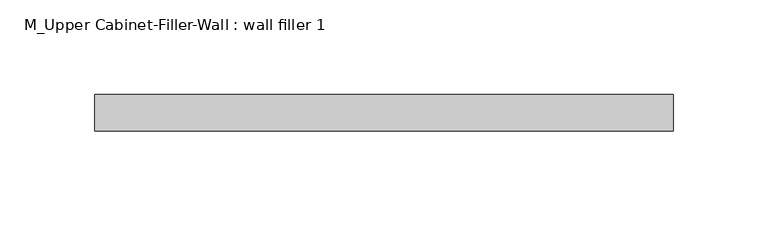
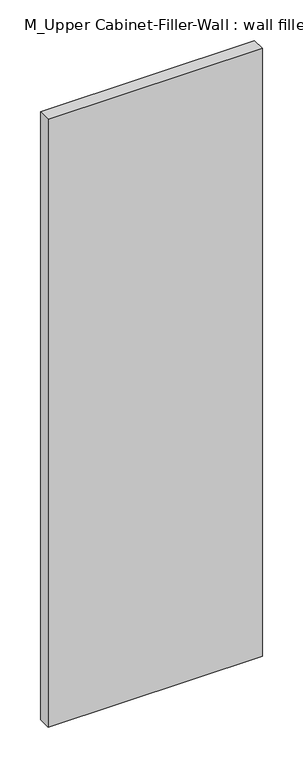
"""IFC4 building model written with IfcOpenShell, lengths in millimetres: furniture geometry, M_Upper Cabinet-Filler-Wall : wall filler 1."""

import ifcopenshell
import ifcopenshell.guid

model = None  # the IFC model being written
_history = None  # IfcOwnerHistory: only IFC2X3 demands one
_inside = {}  # id of a spatial element -> (the spatial element, [elements in it])
_under = {}  # id of a project, library or spatial element -> (it, [spatial elements below it])
_declared = {}  # id of a project -> (the project, [libraries it declares])
_typed = {}  # id of a type object -> (the type object, [elements of that type])
_made_of = {}  # id of a material, layer set ... -> (it, [elements and type objects made of it])


def new_model(schema):
    """Start an empty IFC model of exactly this schema.

    Asked for "IFC4X3", IfcOpenShell would pick the latest addendum, in which some entities
    have other attributes; the version numbers below select the first issue.
    IFC2X3 requires an IfcOwnerHistory on every rooted entity: one is made here for all.
    """
    global model, _history
    if schema == "IFC4X3":
        model = ifcopenshell.file(schema_version=(4, 3, 0, 0))
    else:
        model = ifcopenshell.file(schema=schema)
    _inside.clear()
    _under.clear()
    _declared.clear()
    _typed.clear()
    _made_of.clear()
    _history = None
    if model.schema == "IFC2X3":
        org = make("IfcOrganization", Name="unknown")
        user = make(
            "IfcPersonAndOrganization",
            ThePerson=make("IfcPerson", FamilyName="unknown"),
            TheOrganization=org,
        )
        app = make(
            "IfcApplication",
            ApplicationDeveloper=org,
            Version="unknown",
            ApplicationFullName="unknown",
            ApplicationIdentifier="unknown",
        )
        _history = make(
            "IfcOwnerHistory",
            OwningUser=user,
            OwningApplication=app,
            ChangeAction="ADDED",
            CreationDate=0,
        )
    return model


def make(cls, **values):
    """One entity of the class cls with the attributes given. An attribute that is None is left unset."""
    return model.create_entity(
        cls, **{name: value for name, value in values.items() if value is not None}
    )


def rooted(cls, **values):
    """An entity with a GlobalId (a new one), such as an element, a storey or a relation."""
    return make(cls, GlobalId=ifcopenshell.guid.new(), OwnerHistory=_history, **values)


def si_unit(unit_type, name, prefix=None):
    """IfcSIUnit, for example si_unit("LENGTHUNIT", "METRE", prefix="MILLI")."""
    return make("IfcSIUnit", UnitType=unit_type, Prefix=prefix, Name=name)


def assignment(units):
    """IfcUnitAssignment: the units of a project."""
    return None if units is None else make("IfcUnitAssignment", Units=units)


def point(xyz):
    """IfcCartesianPoint."""
    return None if xyz is None else make("IfcCartesianPoint", Coordinates=xyz)


def direction(xyz):
    """IfcDirection."""
    return None if xyz is None else make("IfcDirection", DirectionRatios=xyz)


def frame(location, z_axis=None, x_axis=None):
    """IfcAxis2Placement3D, a coordinate frame: its origin and axes. An axis left out is left unset."""
    return make(
        "IfcAxis2Placement3D",
        Location=point(location),
        Axis=direction(z_axis),
        RefDirection=direction(x_axis),
    )


def origin():
    """The frame at (0, 0, 0) with its axes left unset."""
    return frame((0.0, 0.0, 0.0))


def place(relative_to, where):
    """IfcLocalPlacement: puts the frame where relative to a parent placement (None: the world)."""
    return make(
        "IfcLocalPlacement", PlacementRelTo=relative_to, RelativePlacement=where
    )


def context(
    kind, dimensions, precision=None, world=None, true_north=None, identifier=None
):
    """IfcGeometricRepresentationContext, for example the 3D "Model" context."""
    return make(
        "IfcGeometricRepresentationContext",
        ContextIdentifier=identifier,
        ContextType=kind,
        CoordinateSpaceDimension=dimensions,
        Precision=precision,
        WorldCoordinateSystem=world,
        TrueNorth=true_north,
    )


def project(units=None, contexts=None):
    """IfcProject with its units and contexts."""
    return rooted(
        "IfcProject",
        Name="project",
        RepresentationContexts=contexts,
        UnitsInContext=assignment(units),
    )


def spatial(cls, under=None, at=None, **own):
    """A site, building, storey or space (cls), placed at a placement, below another one or the project."""
    s = rooted(cls, ObjectPlacement=at, **own)
    if under is not None:
        _under.setdefault(under.id(), (under, []))[1].append(s)
    return s


def polyline(points):
    """IfcPolyline through the points."""
    return make("IfcPolyline", Points=[point(p) for p in points])


def outline(outer, holes=None, kind="AREA"):
    """IfcArbitraryClosedProfileDef: a profile drawn as a closed curve; with holes, ...WithVoids."""
    if holes is None:
        return make("IfcArbitraryClosedProfileDef", ProfileType=kind, OuterCurve=outer)
    return make(
        "IfcArbitraryProfileDefWithVoids",
        ProfileType=kind,
        OuterCurve=outer,
        InnerCurves=holes,
    )


def extrude(swept, where, along, depth):
    """IfcExtrudedAreaSolid: the profile swept, set in the frame where, extruded along a direction by depth."""
    return make(
        "IfcExtrudedAreaSolid",
        SweptArea=swept,
        Position=where,
        ExtrudedDirection=direction(along),
        Depth=depth,
    )


def shape(context_of_items, identifier, shape_type, items):
    """IfcShapeRepresentation: the items that make up one representation, for example the "Body"."""
    return make(
        "IfcShapeRepresentation",
        ContextOfItems=context_of_items,
        RepresentationIdentifier=identifier,
        RepresentationType=shape_type,
        Items=items,
    )


def source(mapping_origin, context_of_items, identifier, shape_type, items):
    """IfcRepresentationMap: a shape defined once, which mapped items show again and again."""
    return make(
        "IfcRepresentationMap",
        MappingOrigin=mapping_origin,
        MappedRepresentation=shape(context_of_items, identifier, shape_type, items),
    )


def transform(
    local_origin,
    x_axis=None,
    y_axis=None,
    z_axis=None,
    scale=None,
    scale2=None,
    scale3=None,
    uniform=True,
):
    """IfcCartesianTransformationOperator3D, or its non-uniform kind. x_axis, y_axis, z_axis: its Axis1, 2, 3."""
    if uniform:
        return make(
            "IfcCartesianTransformationOperator3D",
            Axis1=direction(x_axis),
            Axis2=direction(y_axis),
            LocalOrigin=point(local_origin),
            Scale=scale,
            Axis3=direction(z_axis),
        )
    return make(
        "IfcCartesianTransformationOperator3DnonUniform",
        Axis1=direction(x_axis),
        Axis2=direction(y_axis),
        LocalOrigin=point(local_origin),
        Scale=scale,
        Axis3=direction(z_axis),
        Scale2=scale2,
        Scale3=scale3,
    )


def mapped(mapping_source, mapping_target):
    """IfcMappedItem: shows the shape of a source again, moved by a transform."""
    return make(
        "IfcMappedItem", MappingSource=mapping_source, MappingTarget=mapping_target
    )


def made_of(thing, what):
    """Note that an element or type object is made of a material, layer set ...; save() writes the relation."""
    if what is not None:
        _made_of.setdefault(what.id(), (what, []))[1].append(thing)
    return thing


def element(
    cls,
    number,
    at=None,
    inside=None,
    cuts=None,
    type_object=None,
    material=None,
    context=None,
    identifier="Body",
    shape_type=None,
    held_by="IfcProductDefinitionShape",
    body=None,
    shapes=None,
    **own,
):
    """One element of the class cls, such as IfcWall. Its Tag is "e" and its number.

    at: its placement. inside: the storey or other place that contains it. cuts: it is an
    opening in that element (IfcRelVoidsElement). A single representation is given by context,
    identifier, shape_type and body (its items); several are given by shapes. held_by: the class
    of the entity that holds the representations. save() writes the other relations.
    """
    e = rooted(cls, Tag="e%d" % number, ObjectPlacement=at, **own)
    if body is not None:
        shapes = [shape(context, identifier, shape_type, body)]
    if shapes is not None:
        e.Representation = make(held_by, Representations=shapes)
    if inside is not None:
        _inside.setdefault(inside.id(), (inside, []))[1].append(e)
    if cuts is not None:
        rooted(
            "IfcRelVoidsElement", RelatingBuildingElement=cuts, RelatedOpeningElement=e
        )
    if type_object is not None:
        _typed.setdefault(type_object.id(), (type_object, []))[1].append(e)
    return made_of(e, material)


def aggregate(whole, parts):
    """IfcRelAggregates: a whole, such as a stair, and the parts it consists of."""
    return rooted("IfcRelAggregates", RelatingObject=whole, RelatedObjects=parts)


def save(model, path):
    """Write the relations noted so far, then the file.

    IfcRelAggregates (storeys below a building ...), IfcRelContainedInSpatialStructure (elements
    in a storey), IfcRelDefinesByType, IfcRelAssociatesMaterial and IfcRelDeclares: one each for
    every whole, place, type object, material and project.
    """
    for whole, parts in _under.values():
        aggregate(whole, parts)
    for where, things in _inside.values():
        rooted(
            "IfcRelContainedInSpatialStructure",
            RelatedElements=things,
            RelatingStructure=where,
        )
    for kind, things in _typed.values():
        rooted("IfcRelDefinesByType", RelatedObjects=things, RelatingType=kind)
    for what, things in _made_of.values():
        rooted("IfcRelAssociatesMaterial", RelatedObjects=things, RelatingMaterial=what)
    for by, libraries in _declared.values():
        rooted("IfcRelDeclares", RelatingContext=by, RelatedDefinitions=libraries)
    model.write(path)


def m_upper_cabinet_filler_wall_wall_filler_1_2e82034e(model_context):
    return source(origin(), model_context, "Body", "SweptSolid", [
        extrude(outline(polyline([(-122.6288372, 342.10625), (-122.6288372, 361.15625), (182.1711628, 361.15625), (182.1711628, 342.10625), (-122.6288372, 342.10625)])), frame((0.0, 0.0, 1085.6), z_axis=(0.0, 0.0, 1.0), x_axis=(1.0, 0.0, 0.0)), (0.0, 0.0, 1.0), 914.4),
    ])


if __name__ == "__main__":
    model = new_model("IFC4")
    model_context = context("Model", 3, world=origin())
    ifc_project = project(units=[si_unit("LENGTHUNIT", "METRE", prefix="MILLI")], contexts=[model_context])
    site = spatial("IfcSite", under=ifc_project)
    building = spatial("IfcBuilding", under=site)
    placement = place(None, origin())
    m_upper_cabinet_filler_wall_wall_filler_1_shape = m_upper_cabinet_filler_wall_wall_filler_1_2e82034e(model_context)
    element("IfcFurniture", 1, ObjectType="M_Upper Cabinet-Filler-Wall : wall filler 1", at=placement, inside=building, context=model_context, shape_type="MappedRepresentation", body=[
        mapped(m_upper_cabinet_filler_wall_wall_filler_1_shape, transform((0.0, 0.0, 0.0), x_axis=(1.0, 0.0, 0.0), y_axis=(0.0, 1.0, 0.0), z_axis=(0.0, 0.0, 1.0))),
    ])
    save(model, "model.ifc")

# Revit data of these elements
# Type "M_Upper Cabinet-Filler-Wall : wall filler 1"
#   Depth = 1' - 0"
#   Height = 3' - 0"
#   Top Of Cabinet = 6' - 6.74016"
#   Width = 1' - 0"
#   Cabinet Material = Base cabinet 2120100 Aspekt - 83012120100 - White
#   Default Elevation = 0
# Element 1 (IfcFurniture, "M_Upper Cabinet-Filler-Wall : wall filler 1")
#   Materials on its faces: "Base cabinet 2120100 Aspekt - 83012120100 - White"
# Materials
#   "Base cabinet 2120100 Aspekt - 83012120100 - White": class "Miscellaneous", colour RGB 255 255 255, transparency 0, Manufacturer = "Marbodal", URL = "http://www.marbodal.se", Cost = 0
